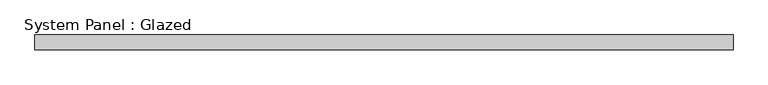
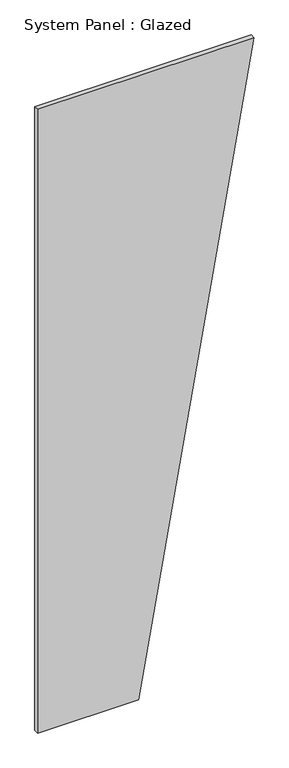
"""IFC4 building model written with IfcOpenShell, lengths in millimetres: plate geometry, System Panel : Glazed."""

from ifc_helpers import new_model, si_unit, frame, origin, place, context, project, spatial, polyline, outline, extrude, source, transform, mapped, element, save


def system_panel_glazed_cd333de7(model_context):
    return source(origin(), model_context, "Body", "SweptSolid", [
        extrude(outline(polyline([(0.0, -601.6711374), (0.0, -40.8082603), (3657.6, 601.6711374), (3657.6, -601.6711374), (0.0, -601.6711374)])), frame((0.0, -44.45, 0.0), z_axis=(0.0, 1.0, 0.0), x_axis=(0.0, 0.0, 1.0)), (0.0, 0.0, 1.0), 25.4),
    ])


if __name__ == "__main__":
    model = new_model("IFC4")
    model_context = context("Model", 3, world=origin())
    ifc_project = project(units=[si_unit("LENGTHUNIT", "METRE", prefix="MILLI")], contexts=[model_context])
    site = spatial("IfcSite", under=ifc_project)
    building = spatial("IfcBuilding", under=site)
    placement = place(None, origin())
    system_panel_glazed_shape = system_panel_glazed_cd333de7(model_context)
    element("IfcPlate", 1, ObjectType="System Panel : Glazed", at=placement, inside=building, context=model_context, shape_type="MappedRepresentation", body=[
        mapped(system_panel_glazed_shape, transform((0.0, 0.0, 0.0), x_axis=(1.0, 0.0, 0.0), y_axis=(0.0, 1.0, 0.0), z_axis=(0.0, 0.0, 1.0))),
    ])
    save(model, "model.ifc")

# Revit data of these elements
# Type "System Panel : Glazed"
#   Construction Type Id = "GSP4R"
#   Analytic Construction = "1/8 in Pilkington single glazing"
#   Visual Light Transmittance = 0.9
#   Solar Heat Gain Coefficient = 0.86
#   Heat Transfer Coefficient (U) = 1.18115 BTU/(h·ft²·°F)
#   Define Thermal Properties by = 1
# Element 1 (IfcPlate, "System Panel : Glazed")
#   Materials on its faces: "Glass"
# Materials
#   "Glass": class "Glass", colour RGB 0 128 192, transparency 0.75, Description = "Soda Lime Glass", Cost = 0
